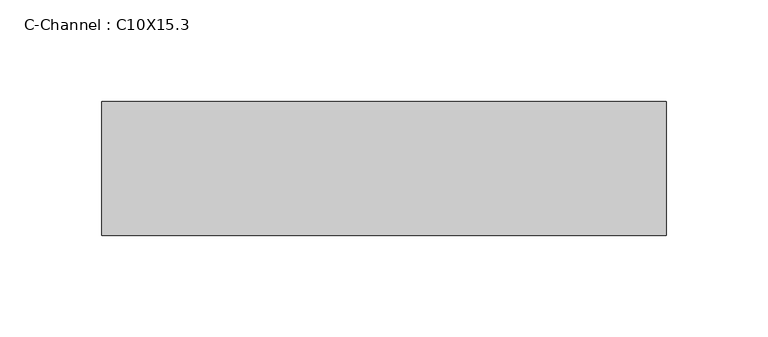
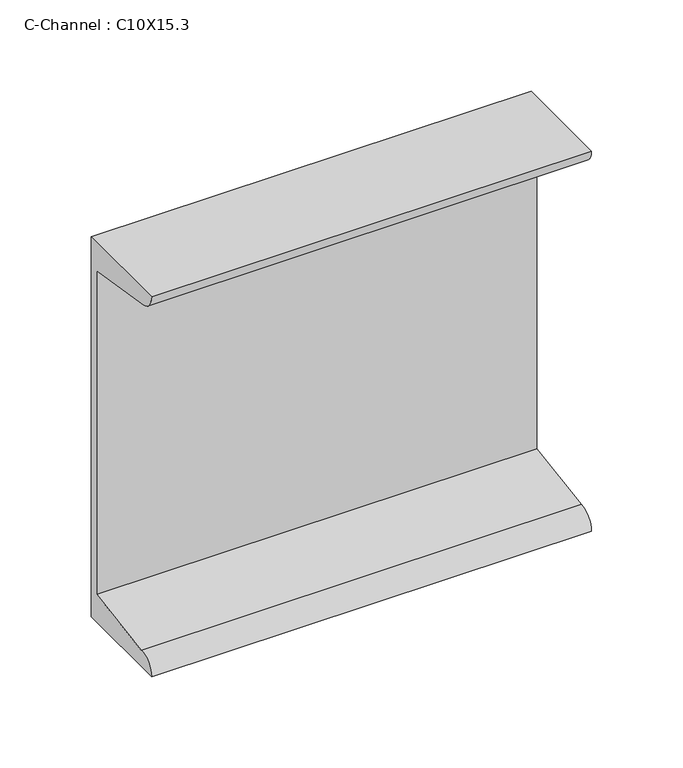
"""IFC4 building model written with IfcOpenShell, lengths in millimetres: beam geometry, C-Channel : C10X15.3."""

from ifc_helpers import new_model, si_unit, point, frame, frame_2d, origin, place, context, project, spatial, polyline, circle_curve, trimmed, segment, composite_curve, outline, extrude, source, transform, mapped, element, save


def c_channel_c10x15_3_72e663a1(model_context):
    return source(origin(), model_context, "Body", "SweptSolid", [
        extrude(outline(composite_curve([segment(polyline([(16.1036, 127.0), (16.1036, -127.0), (-49.9364, -127.0)]), True, "CONTINUOUS"), segment(trimmed(circle_curve(frame_2d((-38.862, -127.0)), 11.0744), [point((-49.9364, -127.0))], [point((-38.862, -115.9256))], False, "CARTESIAN"), True, "CONTINUOUS"), segment(polyline([(-38.862, -115.9256), (10.0076, -108.1854158), (10.0076, 108.1854158), (-38.862, 115.9256)]), True, "CONTINUOUS"), segment(trimmed(circle_curve(frame_2d((-38.862, 127.0)), 11.0744), [point((-38.862, 115.9256))], [point((-49.9364, 127.0))], False, "CARTESIAN"), True, "CONTINUOUS"), segment(polyline([(-49.9364, 127.0), (16.1036, 127.0)]), True, "CONTINUOUS")], self_intersect=False)), frame((-125.73, 0.0, 0.0), z_axis=(1.0, 0.0, 0.0), x_axis=(0.0, 1.0, 0.0)), (0.0, 0.0, 1.0), 278.13),
    ])


if __name__ == "__main__":
    model = new_model("IFC4")
    model_context = context("Model", 3, world=origin())
    ifc_project = project(units=[si_unit("LENGTHUNIT", "METRE", prefix="MILLI")], contexts=[model_context])
    site = spatial("IfcSite", under=ifc_project)
    building = spatial("IfcBuilding", under=site)
    placement = place(None, origin())
    c_channel_c10x15_3_shape = c_channel_c10x15_3_72e663a1(model_context)
    element("IfcBeam", 1, ObjectType="C-Channel : C10X15.3", at=placement, inside=building, context=model_context, shape_type="MappedRepresentation", body=[
        mapped(c_channel_c10x15_3_shape, transform((0.0, 0.0, 0.0), x_axis=(1.0, 0.0, 0.0), y_axis=(0.0, 1.0, 0.0), z_axis=(0.0, 0.0, 1.0))),
    ])
    save(model, "model.ifc")

# Revit data of these elements
# Type "C-Channel : C10X15.3"
#   Assembly Code = "B10"
#   W = 15.3
#   Length [instance default] = 5' - 0"
#   bf = 0' - 2.6"
#   d = 0' - 10"
#   tf = 0' - 0.436"
#   tw = 0' - 0.24"
#   x = 0' - 0.634"
#   A = 0.0311111 SF
#   Structural Material [instance default] = Steel ASTM A36
# Element 1 (IfcBeam, "C-Channel : C10X15.3")
#   Structural Material = Steel ASTM A992
#   Materials on its faces: "Steel ASTM A992"
# Materials
#   "Steel ASTM A36": class "Metal", colour RGB 199 199 199, transparency 0, Description = "Structural steel, ASTM A36 Grade B, mill finish", Cost = 0
#   "Steel ASTM A992": class "Metal", colour RGB 199 199 199, transparency 0, Description = "Structural steel 50ksi", Cost = 0
